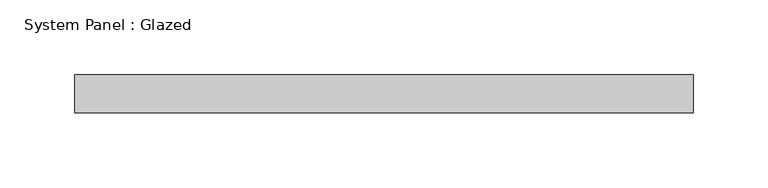
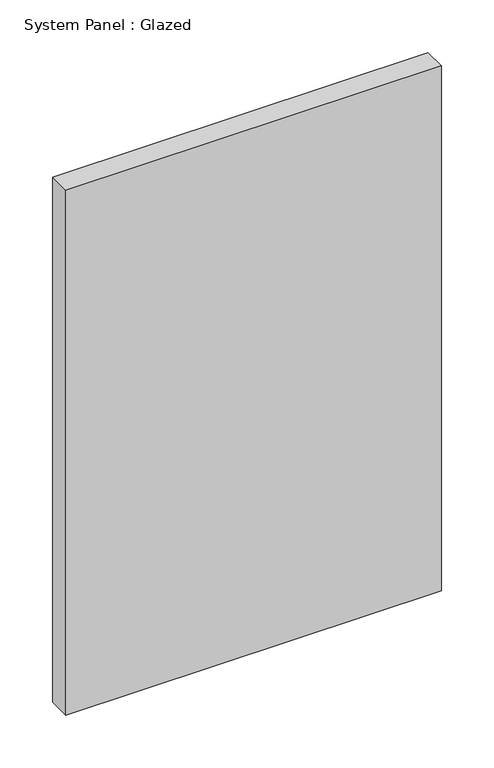
"""IFC4 building model written with IfcOpenShell, lengths in millimetres: plate geometry, System Panel : Glazed."""

from ifc_helpers import new_model, si_unit, origin, origin_with_axes, place, context, project, spatial, polyline, outline, extrude, source, transform, mapped, element, save


def system_panel_glazed_35dff5e5(model_context):
    return source(origin(), model_context, "Body", "SweptSolid", [
        extrude(outline(polyline([(206.3749998, 19.05), (-206.3749998, 19.05), (-206.3749998, 44.45), (206.3749998, 44.45), (206.3749998, 19.05)])), origin_with_axes(), (0.0, 0.0, 1.0), 609.6),
    ])


if __name__ == "__main__":
    model = new_model("IFC4")
    model_context = context("Model", 3, world=origin())
    ifc_project = project(units=[si_unit("LENGTHUNIT", "METRE", prefix="MILLI")], contexts=[model_context])
    site = spatial("IfcSite", under=ifc_project)
    building = spatial("IfcBuilding", under=site)
    placement = place(None, origin())
    system_panel_glazed_shape = system_panel_glazed_35dff5e5(model_context)
    element("IfcPlate", 1, ObjectType="System Panel : Glazed", at=placement, inside=building, context=model_context, shape_type="MappedRepresentation", body=[
        mapped(system_panel_glazed_shape, transform((0.0, 0.0, 0.0), x_axis=(1.0, 0.0, 0.0), y_axis=(0.0, 1.0, 0.0), z_axis=(0.0, 0.0, 1.0))),
    ])
    save(model, "model.ifc")

# Revit data of these elements
# Element 1 (IfcPlate, "System Panel : Glazed")
#   Materials on its faces: "Glass"
# Materials
#   "Glass": class "Glass", colour RGB 0 128 192, transparency 0.75
